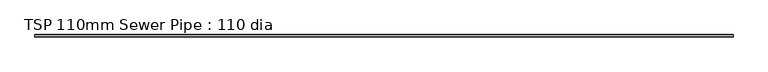
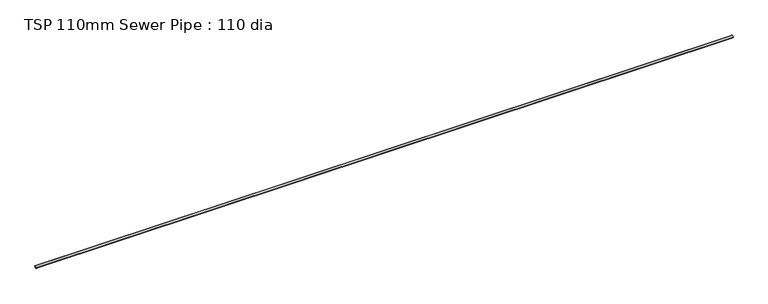
"""IFC4 building model written with IfcOpenShell, lengths in millimetres: flow terminal geometry, TSP 110mm Sewer Pipe : 110 dia."""

from ifc_helpers import new_model, si_unit, point, frame, origin, origin_2d, place, context, project, spatial, circle_curve, trimmed, segment, composite_curve, outline, extrude, source, transform, mapped, element, save


def tsp_110mm_sewer_pipe_110_dia_56459af9(model_context):
    return source(origin(), model_context, "Body", "SweptSolid", [
        extrude(outline(composite_curve([segment(trimmed(circle_curve(origin_2d(), 55.0), [point((-55.0, 0.0))], [point((55.0, 0.0))], False, "CARTESIAN"), True, "CONTINUOUS"), segment(trimmed(circle_curve(origin_2d(), 55.0), [point((55.0, 0.0))], [point((-55.0, 0.0))], False, "CARTESIAN"), True, "CONTINUOUS")], self_intersect=False), holes=[composite_curve([segment(trimmed(circle_curve(origin_2d(), 52.0), [point((-52.0, 0.0))], [point((52.0, 0.0))], True, "CARTESIAN"), True, "CONTINUOUS"), segment(trimmed(circle_curve(origin_2d(), 52.0), [point((52.0, 0.0))], [point((-52.0, 0.0))], True, "CARTESIAN"), True, "CONTINUOUS")], self_intersect=False)]), frame((0.0, 0.0, 0.0), z_axis=(1.0, 0.0, 0.0), x_axis=(0.0, 1.0, 0.0)), (0.0, 0.0, 1.0), 32600.0),
    ])


if __name__ == "__main__":
    model = new_model("IFC4")
    model_context = context("Model", 3, world=origin())
    ifc_project = project(units=[si_unit("LENGTHUNIT", "METRE", prefix="MILLI")], contexts=[model_context])
    site = spatial("IfcSite", under=ifc_project)
    building = spatial("IfcBuilding", under=site)
    placement = place(None, origin())
    tsp_110mm_sewer_pipe_110_dia_shape = tsp_110mm_sewer_pipe_110_dia_56459af9(model_context)
    element("IfcFlowTerminal", 1, ObjectType="TSP 110mm Sewer Pipe : 110 dia", at=placement, inside=building, context=model_context, shape_type="MappedRepresentation", body=[
        mapped(tsp_110mm_sewer_pipe_110_dia_shape, transform((0.0, 0.0, 0.0), x_axis=(1.0, 0.0, 0.0), y_axis=(0.0, 1.0, 0.0), z_axis=(0.0, 0.0, 1.0))),
    ])
    save(model, "model.ifc")

# Revit data of these elements
# Type "TSP 110mm Sewer Pipe : 110 dia"
#   Model = "TSP_110SWB"
#   Model = "TSP_110SWB"
#   Pipe length [instance default] = 1200 mm
#   Pipe dia = 110 mm
#   built-in parameter 1001306 [instance default] = 3.93701 (stored number, unit not read)
#   Default Elevation = 0
# Element 1 (IfcFlowTerminal, "TSP 110mm Sewer Pipe : 110 dia")
#   Pipe length = 32600 mm
#   built-in parameter 1001306 = 106.955 (stored number, unit not read)
#   Materials on its faces: "Laminate, Brown, Matte"
# Materials
#   "Laminate, Brown, Matte": class "Plastic", colour RGB 128 64 0, transparency 0, Description = "Plastic Laminate - Red, Matte", Cost = 0
